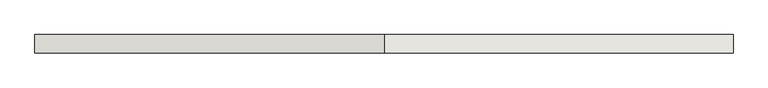
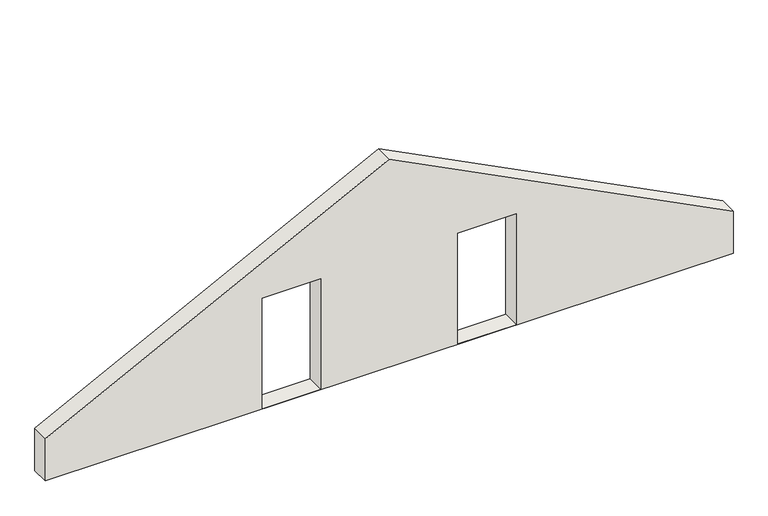
"""IFC4 building model written with IfcOpenShell, lengths in millimetres: wall geometry, 0_3d."""

from ifc_helpers import new_model, si_unit, frame, origin, place, context, project, spatial, polyline, outline, extrude, source, transform, mapped, element, save


def wall_a80c97d2(model_context):
    return source(origin(), model_context, "Body", "SweptSolid", [
        extrude(outline(polyline([(863.3339073, 13300.0), (4251.6781465, 6650.0), (863.3339073, 0.0), (0.0, 0.0), (0.0, 13300.0), (863.3339073, 13300.0)]), holes=[polyline([(10.0, 4190.0), (2270.0, 4190.0), (2270.0, 5325.0), (10.0, 5325.0), (10.0, 4190.0)]), polyline([(10.0, 7975.0), (2270.0, 7975.0), (2270.0, 9110.0), (10.0, 9110.0), (10.0, 7975.0)])]), frame((0.0, 0.0, 0.0), z_axis=(0.0, 1.0, 0.0), x_axis=(0.0, 0.0, 1.0)), (0.0, 0.0, 1.0), 350.0),
    ])


if __name__ == "__main__":
    model = new_model("IFC4")
    model_context = context("Model", 3, world=origin())
    ifc_project = project(units=[si_unit("LENGTHUNIT", "METRE", prefix="MILLI")], contexts=[model_context])
    site = spatial("IfcSite", under=ifc_project)
    building = spatial("IfcBuilding", under=site)
    placement = place(None, origin())
    wall_shape = wall_a80c97d2(model_context)
    element("IfcWall", 1, ObjectType="0_3d", at=placement, inside=building, context=model_context, shape_type="MappedRepresentation", body=[
        mapped(wall_shape, transform((0.0, 0.0, 0.0), x_axis=(1.0, 0.0, 0.0), y_axis=(0.0, 1.0, 0.0), z_axis=(0.0, 0.0, 1.0))),
    ])
    save(model, "model.ifc")

# Revit data of these elements
# Element 1 (IfcWall, "0_3d")
#   Materials on its faces: "holzschalung"
# Materials
#   "holzschalung": class "Unassigned", colour RGB 128 128 128, transparency 0
